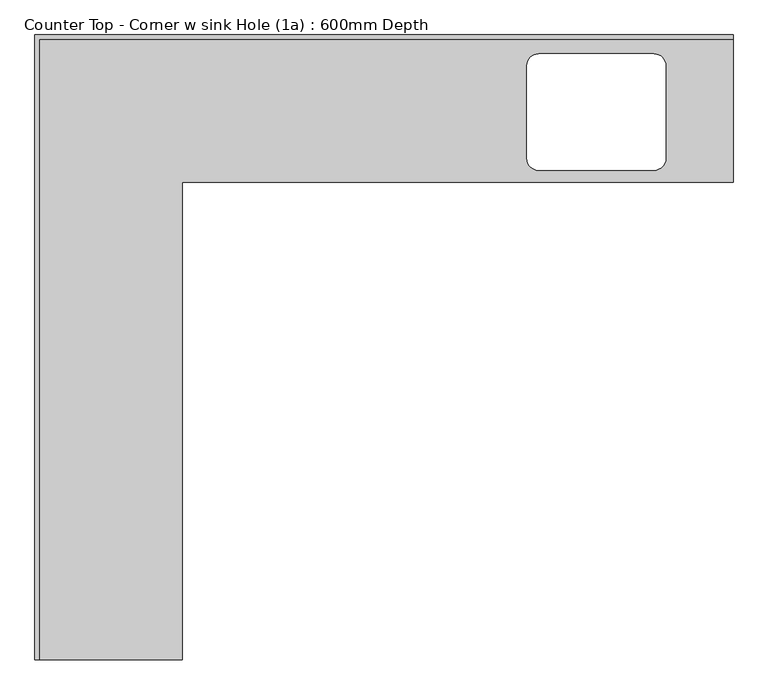
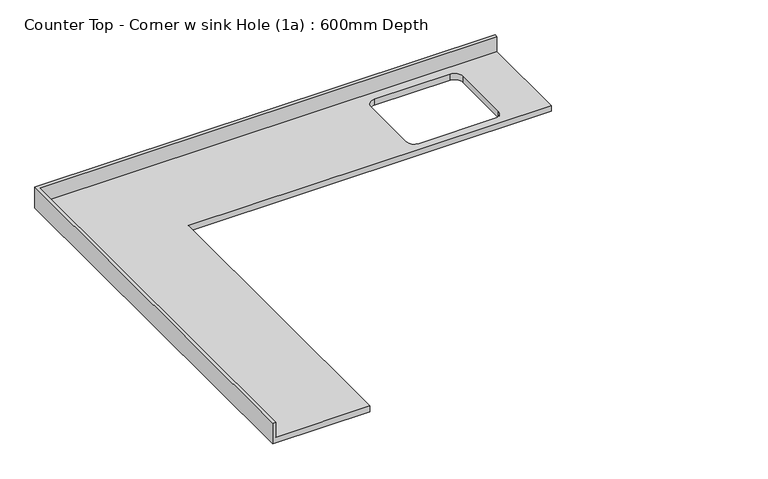
"""IFC4 building model written with IfcOpenShell, lengths in millimetres: furniture geometry, Counter Top - Corner w sink Hole (1a) : 600mm Depth."""

import ifcopenshell
import ifcopenshell.guid

model = None  # the IFC model being written
_history = None  # IfcOwnerHistory: only IFC2X3 demands one
_inside = {}  # id of a spatial element -> (the spatial element, [elements in it])
_under = {}  # id of a project, library or spatial element -> (it, [spatial elements below it])
_declared = {}  # id of a project -> (the project, [libraries it declares])
_typed = {}  # id of a type object -> (the type object, [elements of that type])
_made_of = {}  # id of a material, layer set ... -> (it, [elements and type objects made of it])


def new_model(schema):
    """Start an empty IFC model of exactly this schema.

    Asked for "IFC4X3", IfcOpenShell would pick the latest addendum, in which some entities
    have other attributes; the version numbers below select the first issue.
    IFC2X3 requires an IfcOwnerHistory on every rooted entity: one is made here for all.
    """
    global model, _history
    if schema == "IFC4X3":
        model = ifcopenshell.file(schema_version=(4, 3, 0, 0))
    else:
        model = ifcopenshell.file(schema=schema)
    _inside.clear()
    _under.clear()
    _declared.clear()
    _typed.clear()
    _made_of.clear()
    _history = None
    if model.schema == "IFC2X3":
        org = make("IfcOrganization", Name="unknown")
        user = make(
            "IfcPersonAndOrganization",
            ThePerson=make("IfcPerson", FamilyName="unknown"),
            TheOrganization=org,
        )
        app = make(
            "IfcApplication",
            ApplicationDeveloper=org,
            Version="unknown",
            ApplicationFullName="unknown",
            ApplicationIdentifier="unknown",
        )
        _history = make(
            "IfcOwnerHistory",
            OwningUser=user,
            OwningApplication=app,
            ChangeAction="ADDED",
            CreationDate=0,
        )
    return model


def make(cls, **values):
    """One entity of the class cls with the attributes given. An attribute that is None is left unset."""
    return model.create_entity(
        cls, **{name: value for name, value in values.items() if value is not None}
    )


def rooted(cls, **values):
    """An entity with a GlobalId (a new one), such as an element, a storey or a relation."""
    return make(cls, GlobalId=ifcopenshell.guid.new(), OwnerHistory=_history, **values)


def si_unit(unit_type, name, prefix=None):
    """IfcSIUnit, for example si_unit("LENGTHUNIT", "METRE", prefix="MILLI")."""
    return make("IfcSIUnit", UnitType=unit_type, Prefix=prefix, Name=name)


def assignment(units):
    """IfcUnitAssignment: the units of a project."""
    return None if units is None else make("IfcUnitAssignment", Units=units)


def point(xyz):
    """IfcCartesianPoint."""
    return None if xyz is None else make("IfcCartesianPoint", Coordinates=xyz)


def direction(xyz):
    """IfcDirection."""
    return None if xyz is None else make("IfcDirection", DirectionRatios=xyz)


def frame(location, z_axis=None, x_axis=None):
    """IfcAxis2Placement3D, a coordinate frame: its origin and axes. An axis left out is left unset."""
    return make(
        "IfcAxis2Placement3D",
        Location=point(location),
        Axis=direction(z_axis),
        RefDirection=direction(x_axis),
    )


def origin():
    """The frame at (0, 0, 0) with its axes left unset."""
    return frame((0.0, 0.0, 0.0))


def place(relative_to, where):
    """IfcLocalPlacement: puts the frame where relative to a parent placement (None: the world)."""
    return make(
        "IfcLocalPlacement", PlacementRelTo=relative_to, RelativePlacement=where
    )


def context(
    kind, dimensions, precision=None, world=None, true_north=None, identifier=None
):
    """IfcGeometricRepresentationContext, for example the 3D "Model" context."""
    return make(
        "IfcGeometricRepresentationContext",
        ContextIdentifier=identifier,
        ContextType=kind,
        CoordinateSpaceDimension=dimensions,
        Precision=precision,
        WorldCoordinateSystem=world,
        TrueNorth=true_north,
    )


def project(units=None, contexts=None):
    """IfcProject with its units and contexts."""
    return rooted(
        "IfcProject",
        Name="project",
        RepresentationContexts=contexts,
        UnitsInContext=assignment(units),
    )


def spatial(cls, under=None, at=None, **own):
    """A site, building, storey or space (cls), placed at a placement, below another one or the project."""
    s = rooted(cls, ObjectPlacement=at, **own)
    if under is not None:
        _under.setdefault(under.id(), (under, []))[1].append(s)
    return s


def polyline(points):
    """IfcPolyline through the points."""
    return make("IfcPolyline", Points=[point(p) for p in points])


def circle_curve(where, radius):
    """IfcCircle in the frame where."""
    return make("IfcCircle", Position=where, Radius=radius)


def shape(context_of_items, identifier, shape_type, items):
    """IfcShapeRepresentation: the items that make up one representation, for example the "Body"."""
    return make(
        "IfcShapeRepresentation",
        ContextOfItems=context_of_items,
        RepresentationIdentifier=identifier,
        RepresentationType=shape_type,
        Items=items,
    )


def source(mapping_origin, context_of_items, identifier, shape_type, items):
    """IfcRepresentationMap: a shape defined once, which mapped items show again and again."""
    return make(
        "IfcRepresentationMap",
        MappingOrigin=mapping_origin,
        MappedRepresentation=shape(context_of_items, identifier, shape_type, items),
    )


def transform(
    local_origin,
    x_axis=None,
    y_axis=None,
    z_axis=None,
    scale=None,
    scale2=None,
    scale3=None,
    uniform=True,
):
    """IfcCartesianTransformationOperator3D, or its non-uniform kind. x_axis, y_axis, z_axis: its Axis1, 2, 3."""
    if uniform:
        return make(
            "IfcCartesianTransformationOperator3D",
            Axis1=direction(x_axis),
            Axis2=direction(y_axis),
            LocalOrigin=point(local_origin),
            Scale=scale,
            Axis3=direction(z_axis),
        )
    return make(
        "IfcCartesianTransformationOperator3DnonUniform",
        Axis1=direction(x_axis),
        Axis2=direction(y_axis),
        LocalOrigin=point(local_origin),
        Scale=scale,
        Axis3=direction(z_axis),
        Scale2=scale2,
        Scale3=scale3,
    )


def mapped(mapping_source, mapping_target):
    """IfcMappedItem: shows the shape of a source again, moved by a transform."""
    return make(
        "IfcMappedItem", MappingSource=mapping_source, MappingTarget=mapping_target
    )


def made_of(thing, what):
    """Note that an element or type object is made of a material, layer set ...; save() writes the relation."""
    if what is not None:
        _made_of.setdefault(what.id(), (what, []))[1].append(thing)
    return thing


def element(
    cls,
    number,
    at=None,
    inside=None,
    cuts=None,
    type_object=None,
    material=None,
    context=None,
    identifier="Body",
    shape_type=None,
    held_by="IfcProductDefinitionShape",
    body=None,
    shapes=None,
    **own,
):
    """One element of the class cls, such as IfcWall. Its Tag is "e" and its number.

    at: its placement. inside: the storey or other place that contains it. cuts: it is an
    opening in that element (IfcRelVoidsElement). A single representation is given by context,
    identifier, shape_type and body (its items); several are given by shapes. held_by: the class
    of the entity that holds the representations. save() writes the other relations.
    """
    e = rooted(cls, Tag="e%d" % number, ObjectPlacement=at, **own)
    if body is not None:
        shapes = [shape(context, identifier, shape_type, body)]
    if shapes is not None:
        e.Representation = make(held_by, Representations=shapes)
    if inside is not None:
        _inside.setdefault(inside.id(), (inside, []))[1].append(e)
    if cuts is not None:
        rooted(
            "IfcRelVoidsElement", RelatingBuildingElement=cuts, RelatedOpeningElement=e
        )
    if type_object is not None:
        _typed.setdefault(type_object.id(), (type_object, []))[1].append(e)
    return made_of(e, material)


def aggregate(whole, parts):
    """IfcRelAggregates: a whole, such as a stair, and the parts it consists of."""
    return rooted("IfcRelAggregates", RelatingObject=whole, RelatedObjects=parts)


def save(model, path):
    """Write the relations noted so far, then the file.

    IfcRelAggregates (storeys below a building ...), IfcRelContainedInSpatialStructure (elements
    in a storey), IfcRelDefinesByType, IfcRelAssociatesMaterial and IfcRelDeclares: one each for
    every whole, place, type object, material and project.
    """
    for whole, parts in _under.values():
        aggregate(whole, parts)
    for where, things in _inside.values():
        rooted(
            "IfcRelContainedInSpatialStructure",
            RelatedElements=things,
            RelatingStructure=where,
        )
    for kind, things in _typed.values():
        rooted("IfcRelDefinesByType", RelatedObjects=things, RelatingType=kind)
    for what, things in _made_of.values():
        rooted("IfcRelAssociatesMaterial", RelatedObjects=things, RelatingMaterial=what)
    for by, libraries in _declared.values():
        rooted("IfcRelDeclares", RelatingContext=by, RelatedDefinitions=libraries)
    model.write(path)


def plane_surface(at):
    """IfcPlane: the flat surface through the origin of the frame at, square to its z axis."""
    return make("IfcPlane", Position=at)


def revolved_surface(curve, axis_point, axis_direction):
    """IfcSurfaceOfRevolution: the curve turned about the line through axis_point along axis_direction."""
    return make(
        "IfcSurfaceOfRevolution",
        SweptCurve=make("IfcArbitraryOpenProfileDef", ProfileType="CURVE", Curve=curve),
        AxisPosition=make("IfcAxis1Placement", Location=point(axis_point), Axis=direction(axis_direction)),
    )


def advanced_brep(points, edges, surfaces, faces):
    """IfcAdvancedBrep: a solid bounded by faces that lie on surfaces and meet in shared edges.

    An edge is (start, end): straight between two places in points (the first is 0);
    or (start, end, curve); or (start, end, curve, False) where it runs against its curve.
    A face is (place in surfaces, loops), or (place, loops, False) where it looks against
    its surface's normal. A loop lists edges by number (the first is 1), with a minus sign
    where the edge is run from its end to its start. The first loop is the outer one.
    """
    corners = [point(p) for p in points]
    vertices = [make("IfcVertexPoint", VertexGeometry=c) for c in corners]
    made = []
    for start, end, *more in edges:
        made.append(
            make(
                "IfcEdgeCurve",
                EdgeStart=vertices[start],
                EdgeEnd=vertices[end],
                EdgeGeometry=more[0] if more else make("IfcPolyline", Points=[corners[start], corners[end]]),
                SameSense=more[1] if len(more) > 1 else True,
            )
        )
    hull = []
    for where, loops, *sense in faces:
        bounds = []
        for j, loop in enumerate(loops):
            ring = [make("IfcOrientedEdge", EdgeElement=made[abs(k) - 1], Orientation=k > 0) for k in loop]
            bounds.append(
                make(
                    "IfcFaceOuterBound" if j == 0 else "IfcFaceBound",
                    Bound=make("IfcEdgeLoop", EdgeList=ring),
                    Orientation=True,
                )
            )
        hull.append(make("IfcAdvancedFace", Bounds=bounds, FaceSurface=surfaces[where], SameSense=sense[0] if sense else True))
    return make("IfcAdvancedBrep", Outer=make("IfcClosedShell", CfsFaces=hull))


def counter_top_corner_w_sink_hole_1a_600mm_depth_949058ad(model_context):
    return source(origin(), model_context, "Body", "AdvancedBrep", [
        advanced_brep(
        [(-575.4622951, -2650.0, 900.0), (-575.4622951, -625.0, 900.0), (1760.5377049, -625.0, 900.0), (1760.5377049, -19.05, 900.0), (-1181.4122951, -19.05, 900.0), (-1181.4122951, -2650.0, 900.0), (1424.9847176, -80.9334893, 900.0), (1474.9847176, -130.9334893, 900.0), (1474.9847176, -524.5706264, 900.0), (1424.9847176, -574.5706264, 900.0), (936.4146442, -574.5706264, 900.0), (886.4146442, -524.5706264, 900.0), (886.4146442, -130.9334893, 900.0), (936.4146442, -80.9334893, 900.0), (1760.5377049, 0.0, 860.0), (1760.5377049, -625.0, 860.0), (-575.4622951, -625.0, 860.0), (-575.4622951, -2650.0, 860.0), (-1200.4622951, -2650.0, 860.0), (-1200.4622951, 0.0, 860.0), (1424.9847176, -80.9334893, 860.0), (936.4146442, -80.9334893, 860.0), (886.4146442, -130.9334893, 860.0), (886.4146442, -524.5706264, 860.0), (936.4146442, -574.5706264, 860.0), (1424.9847176, -574.5706264, 860.0), (1474.9847176, -524.5706264, 860.0), (1474.9847176, -130.9334893, 860.0), (-1200.4622951, 0.0, 1001.6), (1760.5377049, 0.0, 1001.6), (-1200.4622951, -2650.0, 1001.6), (-1181.4122951, -2650.0, 1001.6), (1760.5377049, -19.05, 1001.6), (-1181.4122951, -19.05, 1001.6)],
        [
            (0, 1),
            (1, 2),
            (2, 3),
            (3, 4),
            (4, 5),
            (5, 0),
            (6, 7, circle_curve(frame((1424.9847176, -130.9334893, 900.0), z_axis=(0.0, 0.0, -1.0), x_axis=(1.0, 0.0, 0.0)), 50.0)),
            (7, 8),
            (8, 9, circle_curve(frame((1424.9847176, -524.5706264, 900.0), z_axis=(0.0, 0.0, -1.0), x_axis=(1.0, 0.0, 0.0)), 50.0)),
            (9, 10),
            (10, 11, circle_curve(frame((936.4146442, -524.5706264, 900.0), z_axis=(0.0, 0.0, -1.0), x_axis=(1.0, 0.0, 0.0)), 50.0)),
            (11, 12),
            (12, 13, circle_curve(frame((936.4146442, -130.9334893, 900.0), z_axis=(0.0, 0.0, -1.0), x_axis=(1.0, 0.0, 0.0)), 50.0)),
            (13, 6),
            (14, 15),
            (15, 16),
            (16, 17),
            (17, 18),
            (18, 19),
            (19, 14),
            (20, 21),
            (21, 22, circle_curve(frame((936.4146442, -130.9334893, 860.0), z_axis=(0.0, 0.0, 1.0), x_axis=(1.0, 0.0, 0.0)), 50.0)),
            (22, 23),
            (23, 24, circle_curve(frame((936.4146442, -524.5706264, 860.0), z_axis=(0.0, 0.0, 1.0), x_axis=(1.0, 0.0, 0.0)), 50.0)),
            (24, 25),
            (25, 26, circle_curve(frame((1424.9847176, -524.5706264, 860.0), z_axis=(0.0, 0.0, 1.0), x_axis=(1.0, 0.0, 0.0)), 50.0)),
            (26, 27),
            (27, 20, circle_curve(frame((1424.9847176, -130.9334893, 860.0), z_axis=(0.0, 0.0, 1.0), x_axis=(1.0, 0.0, 0.0)), 50.0)),
            (19, 28),
            (28, 29),
            (29, 14),
            (18, 30),
            (30, 28),
            (17, 0),
            (5, 31),
            (31, 30),
            (16, 1),
            (15, 2),
            (29, 32),
            (32, 3),
            (6, 20),
            (27, 7),
            (26, 8),
            (25, 9),
            (24, 10),
            (23, 11),
            (22, 12),
            (21, 13),
            (31, 33),
            (33, 32),
            (33, 4),
        ],
        [
            plane_surface(frame((-1200.4622951, 0.0, 900.0), z_axis=(0.0, 0.0, 1.0), x_axis=(-1.0, 0.0, 0.0))),
            plane_surface(frame((-1200.4622951, 0.0, 860.0), z_axis=(0.0, 0.0, -1.0), x_axis=(1.0, 0.0, 0.0))),
            plane_surface(frame((1760.5377049, 0.0, 900.0), z_axis=(0.0, 1.0, 0.0), x_axis=(0.0, 0.0, -1.0))),
            plane_surface(frame((-1200.4622951, 0.0, 900.0), z_axis=(-1.0, 0.0, 0.0), x_axis=(0.0, 0.0, -1.0))),
            plane_surface(frame((-1200.4622951, -2650.0, 900.0), z_axis=(0.0, -1.0, 0.0), x_axis=(0.0, 0.0, -1.0))),
            plane_surface(frame((-575.4622951, -2650.0, 900.0), z_axis=(1.0, 0.0, 0.0), x_axis=(0.0, 0.0, -1.0))),
            plane_surface(frame((-575.4622951, -625.0, 900.0), z_axis=(0.0, -1.0, 0.0), x_axis=(0.0, 0.0, -1.0))),
            plane_surface(frame((1760.5377049, -625.0, 900.0), z_axis=(1.0, 0.0, 0.0), x_axis=(0.0, 0.0, -1.0))),
            revolved_surface(polyline([(1474.9847176, -130.9334893, 860.0), (1474.9847176, -130.9334893, 900.0)]), (1424.9847176, -130.9334893, 0.0), (0.0, 0.0, -1.0)),
            plane_surface(frame((1474.9847176, -130.9334893, 900.0), z_axis=(-1.0, 0.0, 0.0), x_axis=(0.0, 0.0, -1.0))),
            revolved_surface(polyline([(1474.9847176, -524.5706264, 860.0), (1474.9847176, -524.5706264, 900.0)]), (1424.9847176, -524.5706264, 0.0), (0.0, 0.0, -1.0)),
            plane_surface(frame((1424.9847176, -574.5706264, 900.0), z_axis=(0.0, 1.0, 0.0), x_axis=(0.0, 0.0, -1.0))),
            revolved_surface(polyline([(986.4146442, -524.5706264, 860.0), (986.4146442, -524.5706264, 900.0)]), (936.4146442, -524.5706264, 0.0), (0.0, 0.0, -1.0)),
            plane_surface(frame((886.4146442, -524.5706264, 900.0), z_axis=(1.0, 0.0, 0.0), x_axis=(0.0, 0.0, -1.0))),
            revolved_surface(polyline([(986.4146442, -130.9334893, 860.0), (986.4146442, -130.9334893, 900.0)]), (936.4146442, -130.9334893, 0.0), (0.0, 0.0, -1.0)),
            plane_surface(frame((936.4146442, -80.9334893, 900.0), z_axis=(0.0, -1.0, 0.0), x_axis=(0.0, 0.0, -1.0))),
            plane_surface(frame((-1200.4622951, 0.0, 1001.6), z_axis=(0.0, 0.0, 1.0), x_axis=(0.0, -1.0, 0.0))),
            plane_surface(frame((-1200.4622951, -19.05, 1001.6), z_axis=(0.0, -1.0, 0.0), x_axis=(0.0, 0.0, -1.0))),
            plane_surface(frame((-1181.4122951, -2650.0, 1001.6), z_axis=(1.0, 0.0, 0.0), x_axis=(0.0, 0.0, -1.0))),
        ],
        [
            (0, [[1, 2, 3, 4, 5, 6], [7, 8, 9, 10, 11, 12, 13, 14]]),
            (1, [[15, 16, 17, 18, 19, 20], [21, 22, 23, 24, 25, 26, 27, 28]]),
            (2, [[-20, 29, 30, 31]]),
            (3, [[-19, 32, 33, -29]]),
            (4, [[-32, -18, 34, -6, 35, 36]]),
            (5, [[-1, -34, -17, 37]]),
            (6, [[-2, -37, -16, 38]]),
            (7, [[-15, -31, 39, 40, -3, -38]]),
            (8, [[-7, 41, -28, 42]]),
            (9, [[-8, -42, -27, 43]]),
            (10, [[-9, -43, -26, 44]]),
            (11, [[-10, -44, -25, 45]]),
            (12, [[-11, -45, -24, 46]]),
            (13, [[-12, -46, -23, 47]]),
            (14, [[-13, -47, -22, 48]]),
            (15, [[-14, -48, -21, -41]]),
            (16, [[-33, -36, 49, 50, -39, -30]]),
            (17, [[-40, -50, 51, -4]]),
            (18, [[-49, -35, -5, -51]]),
        ],
    ),
    ])


if __name__ == "__main__":
    model = new_model("IFC4")
    model_context = context("Model", 3, world=origin())
    ifc_project = project(units=[si_unit("LENGTHUNIT", "METRE", prefix="MILLI")], contexts=[model_context])
    site = spatial("IfcSite", under=ifc_project)
    building = spatial("IfcBuilding", under=site)
    placement = place(None, origin())
    counter_top_corner_w_sink_hole_1a_600mm_depth_shape = counter_top_corner_w_sink_hole_1a_600mm_depth_949058ad(model_context)
    element("IfcFurniture", 1, ObjectType="Counter Top - Corner w sink Hole (1a) : 600mm Depth", at=placement, inside=building, context=model_context, shape_type="MappedRepresentation", body=[
        mapped(counter_top_corner_w_sink_hole_1a_600mm_depth_shape, transform((0.0, 0.0, 0.0), x_axis=(1.0, 0.0, 0.0), y_axis=(0.0, 1.0, 0.0), z_axis=(0.0, 0.0, 1.0))),
    ])
    save(model, "model.ifc")

# Revit data of these elements
# Project information
#   Project Status = "Project Status"
#   Client Name = "Revit Project"
#   Project Address = "Enter address here"
#   Project Name = "Two Storey Residence"
#   Project Number = "RARC01"
# Type "Counter Top - Corner w sink Hole (1a) : 600mm Depth"
#   Keynote = "N10"
#   Width = 625 mm
#   Counter Thickness = 40 mm
#   Depth = 625 mm
#   Height = 900 mm
#   Length - Leg 1 [instance default] = 2250 mm
#   Length - Leg 2 [instance default] = 2150 mm
#   Sink Location [instance default] = 1100 mm
#   Sink Location To Wall [instance default] = 150 mm
#   Sink Opening Depth [instance default] = 380 mm
#   Sink Opening Width [instance default] = 585 mm
#   Vis - Worktop Upstand = yes
#   Material Worktop = Laminate - Marble
#   Default Elevation = 0
# Element 1 (IfcFurniture, "Counter Top - Corner w sink Hole (1a) : 600mm Depth")
#   Length - Leg 1 = 2961 mm
#   Length - Leg 2 = 2650 mm
#   Sink Location = 2086.877 mm
#   Sink Location To Wall = 80.933 mm
#   Sink Opening Depth = 493.637 mm
#   Sink Opening Width = 588.57 mm
#   Materials on its faces: "Laminate - Marble"
# Materials
#   "Laminate - Marble": class "Miscellaneous", colour RGB 196 174 157, transparency 0
